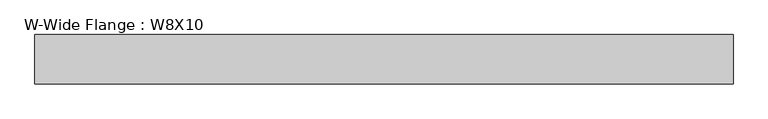
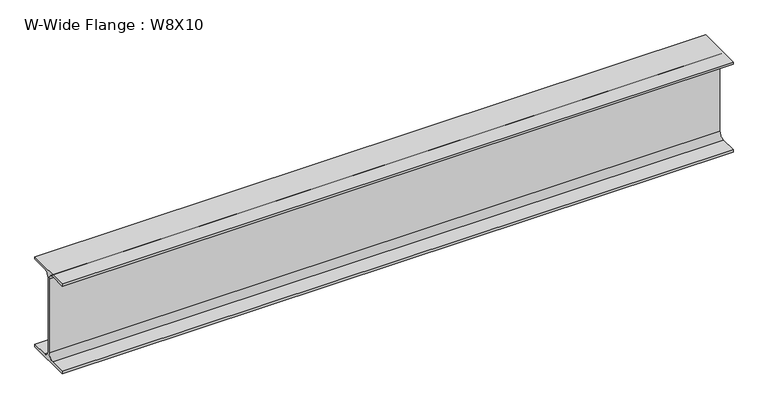
"""IFC4 building model written with IfcOpenShell, lengths in millimetres: beam geometry, W-Wide Flange : W8X10."""

from ifc_helpers import new_model, si_unit, point, frame, frame_2d, origin, place, context, project, spatial, polyline, circle_curve, trimmed, segment, composite_curve, outline, extrude, source, transform, mapped, element, save


def w_wide_flange_w8x10_f6404ef0(model_context):
    return source(origin(), model_context, "Body", "SweptSolid", [
        extrude(outline(composite_curve([segment(polyline([(50.038, -94.996), (50.038, -100.203), (-50.038, -100.203), (-50.038, -94.996), (-14.4145, -94.996)]), True, "CONTINUOUS"), segment(trimmed(circle_curve(frame_2d((-14.4145, -82.7405)), 12.2555), [point((-14.4145, -94.996))], [point((-2.159, -82.7405))], True, "CARTESIAN"), True, "CONTINUOUS"), segment(polyline([(-2.159, -82.7405), (-2.159, 82.7405)]), True, "CONTINUOUS"), segment(trimmed(circle_curve(frame_2d((-14.4145, 82.7405)), 12.2555), [point((-2.159, 82.7405))], [point((-14.4145, 94.996))], True, "CARTESIAN"), True, "CONTINUOUS"), segment(polyline([(-14.4145, 94.996), (-50.038, 94.996), (-50.038, 100.203), (50.038, 100.203), (50.038, 94.996), (14.4145, 94.996)]), True, "CONTINUOUS"), segment(trimmed(circle_curve(frame_2d((14.4145, 82.7405)), 12.2555), [point((14.4145, 94.996))], [point((2.159, 82.7405))], True, "CARTESIAN"), True, "CONTINUOUS"), segment(polyline([(2.159, 82.7405), (2.159, -82.7405)]), True, "CONTINUOUS"), segment(trimmed(circle_curve(frame_2d((14.4145, -82.7405)), 12.2555), [point((2.159, -82.7405))], [point((14.4145, -94.996))], True, "CARTESIAN"), True, "CONTINUOUS"), segment(polyline([(14.4145, -94.996), (50.038, -94.996)]), True, "CONTINUOUS")], self_intersect=False)), frame((-697.1605469, 0.0, 0.0), z_axis=(1.0, 0.0, 0.0), x_axis=(0.0, 1.0, 0.0)), (0.0, 0.0, 1.0), 1413.1230469),
    ])


if __name__ == "__main__":
    model = new_model("IFC4")
    model_context = context("Model", 3, world=origin())
    ifc_project = project(units=[si_unit("LENGTHUNIT", "METRE", prefix="MILLI")], contexts=[model_context])
    site = spatial("IfcSite", under=ifc_project)
    building = spatial("IfcBuilding", under=site)
    placement = place(None, origin())
    w_wide_flange_w8x10_shape = w_wide_flange_w8x10_f6404ef0(model_context)
    element("IfcBeam", 1, ObjectType="W-Wide Flange : W8X10", at=placement, inside=building, context=model_context, shape_type="MappedRepresentation", body=[
        mapped(w_wide_flange_w8x10_shape, transform((0.0, 0.0, 0.0), x_axis=(1.0, 0.0, 0.0), y_axis=(0.0, 1.0, 0.0), z_axis=(0.0, 0.0, 1.0))),
    ])
    save(model, "model.ifc")

# Revit data of these elements
# Type "W-Wide Flange : W8X10"
#   Assembly Code = "B10"
#   W = 10
#   Length [instance default] = 1524 mm
#   bf = 100.076 mm
#   d = 200.406 mm
#   k = 17.463 mm
#   k2 = 12.255 mm
#   tf = 5.207 mm
#   tw = 4.318 mm
#   A = 0.00190967 m²
#   Structural Material [instance default] = Steel ASTM A992
# Element 1 (IfcBeam, "W-Wide Flange : W8X10")
#   Structural Material = Aluminum, Anodized Red
#   Materials on its faces: "Aluminum, Anodized Red"
# Materials
#   "Steel ASTM A992": class "Metal", colour RGB 128 0 0, transparency 0, Description = "Structural steel 50ksi", Cost = 0
#   "Aluminum, Anodized Red": class "Metal", colour RGB 120 120 120, transparency 0, Description = "Anodized aluminum, red", Cost = 0
